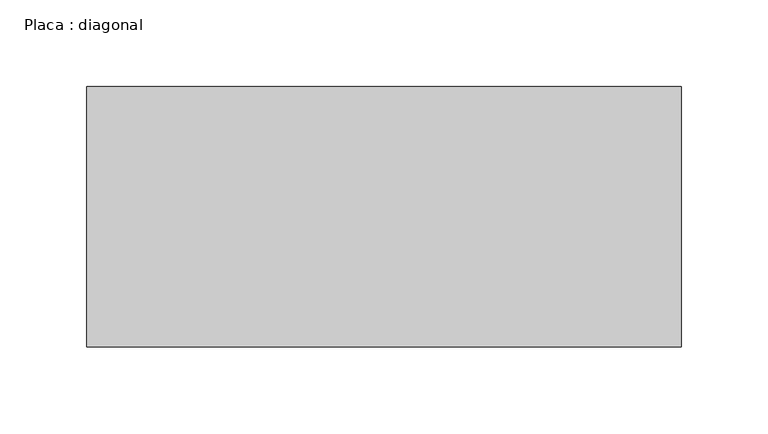
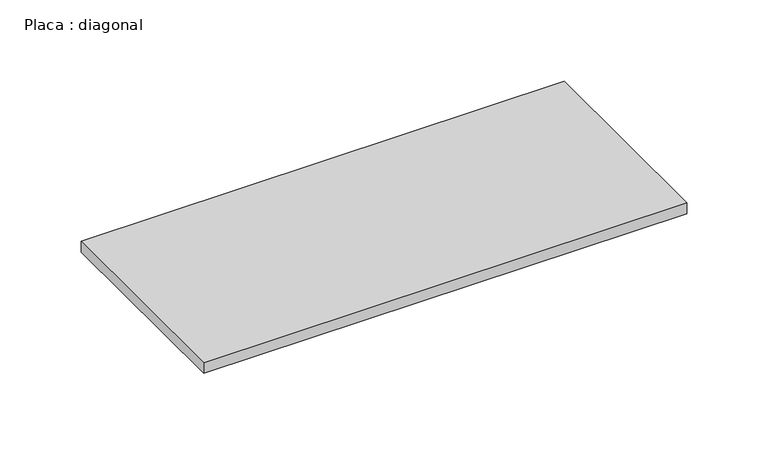
"""IFC4 building model written with IfcOpenShell, lengths in millimetres: beam geometry, Placa : diagonal."""

from ifc_helpers import new_model, si_unit, frame, origin, place, context, project, spatial, polyline, outline, extrude, source, transform, mapped, element, save


def placa_diagonal_cac56629(model_context):
    return source(origin(), model_context, "Body", "SweptSolid", [
        extrude(outline(polyline([(171.6122413, 75.0), (171.6122413, -75.0), (-170.6977781, -75.0), (-170.6977781, 75.0), (171.6122413, 75.0)])), frame((0.0, 0.0, -4.0), z_axis=(0.0, 0.0, 1.0), x_axis=(1.0, 0.0, 0.0)), (0.0, 0.0, 1.0), 8.0),
    ])


if __name__ == "__main__":
    model = new_model("IFC4")
    model_context = context("Model", 3, world=origin())
    ifc_project = project(units=[si_unit("LENGTHUNIT", "METRE", prefix="MILLI")], contexts=[model_context])
    site = spatial("IfcSite", under=ifc_project)
    building = spatial("IfcBuilding", under=site)
    placement = place(None, origin())
    placa_diagonal_shape = placa_diagonal_cac56629(model_context)
    element("IfcBeam", 1, ObjectType="Placa : diagonal", at=placement, inside=building, context=model_context, shape_type="MappedRepresentation", body=[
        mapped(placa_diagonal_shape, transform((0.0, 0.0, 0.0), x_axis=(1.0, 0.0, 0.0), y_axis=(0.0, 1.0, 0.0), z_axis=(0.0, 0.0, 1.0))),
    ])
    save(model, "model.ifc")

# Revit data of these elements
# Type "Placa : diagonal"
#   W = 0
#   Length [instance default] = 1.50 m
#   b = 0.15 m
#   d = 0.008 m
#   A = 0 m²
#   Structural Material [instance default] = Aço, 45-345
# Element 1 (IfcBeam, "Placa : diagonal")
#   Materials on its faces: "Aço, 45-345"
# Materials
#   "Aço, 45-345": class "Metal", colour RGB 247 247 247, transparency 0, Description = "Aço 345 MPa", Cost = 0
